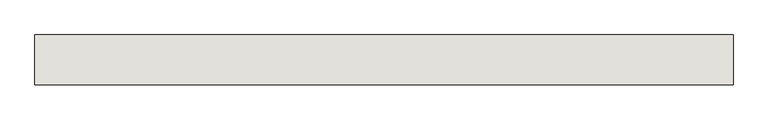
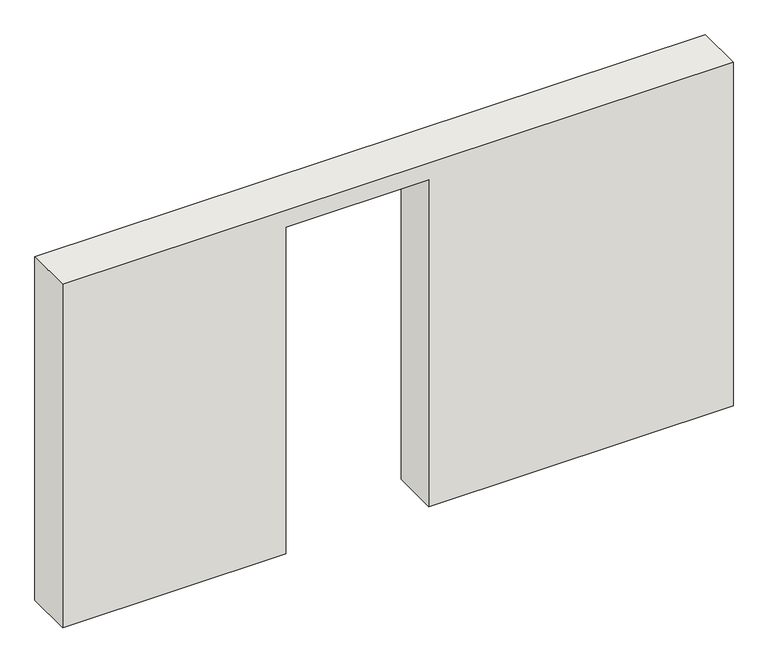
"""IFC4 building model written with IfcOpenShell, lengths in millimetres: wall geometry, 0_3d."""

from ifc_helpers import new_model, si_unit, frame, origin, place, context, project, spatial, polyline, outline, extrude, source, transform, mapped, element, save


def wall_4a9c532f(model_context):
    return source(origin(), model_context, "Body", "SweptSolid", [
        extrude(outline(polyline([(2740.0, 2905.0), (0.0, 2905.0), (0.0, 5320.0), (2880.0, 5320.0), (2880.0, 0.0), (0.0, 0.0), (0.0, 1770.0), (2740.0, 1770.0), (2740.0, 2905.0)])), frame((0.0, 0.0, 0.0), z_axis=(0.0, 1.0, 0.0), x_axis=(0.0, 0.0, 1.0)), (0.0, 0.0, 1.0), 380.0),
    ])


if __name__ == "__main__":
    model = new_model("IFC4")
    model_context = context("Model", 3, world=origin())
    ifc_project = project(units=[si_unit("LENGTHUNIT", "METRE", prefix="MILLI")], contexts=[model_context])
    site = spatial("IfcSite", under=ifc_project)
    building = spatial("IfcBuilding", under=site)
    placement = place(None, origin())
    wall_shape = wall_4a9c532f(model_context)
    element("IfcWall", 1, ObjectType="0_3d", at=placement, inside=building, context=model_context, shape_type="MappedRepresentation", body=[
        mapped(wall_shape, transform((0.0, 0.0, 0.0), x_axis=(1.0, 0.0, 0.0), y_axis=(0.0, 1.0, 0.0), z_axis=(0.0, 0.0, 1.0))),
    ])
    save(model, "model.ifc")

# Revit data of these elements
# Element 1 (IfcWall, "0_3d")
#   Materials on its faces: "holzschalung"
# Materials
#   "holzschalung": class "Unassigned", colour RGB 128 128 128, transparency 0
